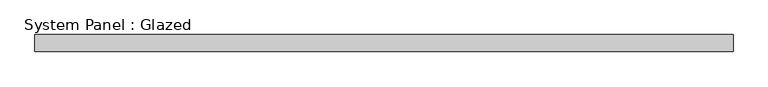
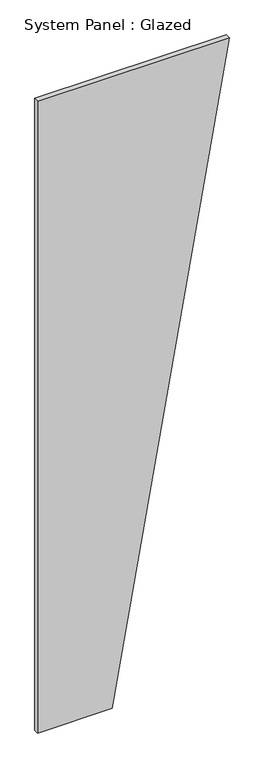
"""IFC4 building model written with IfcOpenShell, lengths in millimetres: plate geometry, System Panel : Glazed."""

import ifcopenshell
import ifcopenshell.guid

model = None  # the IFC model being written
_history = None  # IfcOwnerHistory: only IFC2X3 demands one
_inside = {}  # id of a spatial element -> (the spatial element, [elements in it])
_under = {}  # id of a project, library or spatial element -> (it, [spatial elements below it])
_declared = {}  # id of a project -> (the project, [libraries it declares])
_typed = {}  # id of a type object -> (the type object, [elements of that type])
_made_of = {}  # id of a material, layer set ... -> (it, [elements and type objects made of it])


def new_model(schema):
    """Start an empty IFC model of exactly this schema.

    Asked for "IFC4X3", IfcOpenShell would pick the latest addendum, in which some entities
    have other attributes; the version numbers below select the first issue.
    IFC2X3 requires an IfcOwnerHistory on every rooted entity: one is made here for all.
    """
    global model, _history
    if schema == "IFC4X3":
        model = ifcopenshell.file(schema_version=(4, 3, 0, 0))
    else:
        model = ifcopenshell.file(schema=schema)
    _inside.clear()
    _under.clear()
    _declared.clear()
    _typed.clear()
    _made_of.clear()
    _history = None
    if model.schema == "IFC2X3":
        org = make("IfcOrganization", Name="unknown")
        user = make(
            "IfcPersonAndOrganization",
            ThePerson=make("IfcPerson", FamilyName="unknown"),
            TheOrganization=org,
        )
        app = make(
            "IfcApplication",
            ApplicationDeveloper=org,
            Version="unknown",
            ApplicationFullName="unknown",
            ApplicationIdentifier="unknown",
        )
        _history = make(
            "IfcOwnerHistory",
            OwningUser=user,
            OwningApplication=app,
            ChangeAction="ADDED",
            CreationDate=0,
        )
    return model


def make(cls, **values):
    """One entity of the class cls with the attributes given. An attribute that is None is left unset."""
    return model.create_entity(
        cls, **{name: value for name, value in values.items() if value is not None}
    )


def rooted(cls, **values):
    """An entity with a GlobalId (a new one), such as an element, a storey or a relation."""
    return make(cls, GlobalId=ifcopenshell.guid.new(), OwnerHistory=_history, **values)


def si_unit(unit_type, name, prefix=None):
    """IfcSIUnit, for example si_unit("LENGTHUNIT", "METRE", prefix="MILLI")."""
    return make("IfcSIUnit", UnitType=unit_type, Prefix=prefix, Name=name)


def assignment(units):
    """IfcUnitAssignment: the units of a project."""
    return None if units is None else make("IfcUnitAssignment", Units=units)


def point(xyz):
    """IfcCartesianPoint."""
    return None if xyz is None else make("IfcCartesianPoint", Coordinates=xyz)


def direction(xyz):
    """IfcDirection."""
    return None if xyz is None else make("IfcDirection", DirectionRatios=xyz)


def frame(location, z_axis=None, x_axis=None):
    """IfcAxis2Placement3D, a coordinate frame: its origin and axes. An axis left out is left unset."""
    return make(
        "IfcAxis2Placement3D",
        Location=point(location),
        Axis=direction(z_axis),
        RefDirection=direction(x_axis),
    )


def origin():
    """The frame at (0, 0, 0) with its axes left unset."""
    return frame((0.0, 0.0, 0.0))


def place(relative_to, where):
    """IfcLocalPlacement: puts the frame where relative to a parent placement (None: the world)."""
    return make(
        "IfcLocalPlacement", PlacementRelTo=relative_to, RelativePlacement=where
    )


def context(
    kind, dimensions, precision=None, world=None, true_north=None, identifier=None
):
    """IfcGeometricRepresentationContext, for example the 3D "Model" context."""
    return make(
        "IfcGeometricRepresentationContext",
        ContextIdentifier=identifier,
        ContextType=kind,
        CoordinateSpaceDimension=dimensions,
        Precision=precision,
        WorldCoordinateSystem=world,
        TrueNorth=true_north,
    )


def project(units=None, contexts=None):
    """IfcProject with its units and contexts."""
    return rooted(
        "IfcProject",
        Name="project",
        RepresentationContexts=contexts,
        UnitsInContext=assignment(units),
    )


def spatial(cls, under=None, at=None, **own):
    """A site, building, storey or space (cls), placed at a placement, below another one or the project."""
    s = rooted(cls, ObjectPlacement=at, **own)
    if under is not None:
        _under.setdefault(under.id(), (under, []))[1].append(s)
    return s


def polyline(points):
    """IfcPolyline through the points."""
    return make("IfcPolyline", Points=[point(p) for p in points])


def outline(outer, holes=None, kind="AREA"):
    """IfcArbitraryClosedProfileDef: a profile drawn as a closed curve; with holes, ...WithVoids."""
    if holes is None:
        return make("IfcArbitraryClosedProfileDef", ProfileType=kind, OuterCurve=outer)
    return make(
        "IfcArbitraryProfileDefWithVoids",
        ProfileType=kind,
        OuterCurve=outer,
        InnerCurves=holes,
    )


def extrude(swept, where, along, depth):
    """IfcExtrudedAreaSolid: the profile swept, set in the frame where, extruded along a direction by depth."""
    return make(
        "IfcExtrudedAreaSolid",
        SweptArea=swept,
        Position=where,
        ExtrudedDirection=direction(along),
        Depth=depth,
    )


def shape(context_of_items, identifier, shape_type, items):
    """IfcShapeRepresentation: the items that make up one representation, for example the "Body"."""
    return make(
        "IfcShapeRepresentation",
        ContextOfItems=context_of_items,
        RepresentationIdentifier=identifier,
        RepresentationType=shape_type,
        Items=items,
    )


def source(mapping_origin, context_of_items, identifier, shape_type, items):
    """IfcRepresentationMap: a shape defined once, which mapped items show again and again."""
    return make(
        "IfcRepresentationMap",
        MappingOrigin=mapping_origin,
        MappedRepresentation=shape(context_of_items, identifier, shape_type, items),
    )


def transform(
    local_origin,
    x_axis=None,
    y_axis=None,
    z_axis=None,
    scale=None,
    scale2=None,
    scale3=None,
    uniform=True,
):
    """IfcCartesianTransformationOperator3D, or its non-uniform kind. x_axis, y_axis, z_axis: its Axis1, 2, 3."""
    if uniform:
        return make(
            "IfcCartesianTransformationOperator3D",
            Axis1=direction(x_axis),
            Axis2=direction(y_axis),
            LocalOrigin=point(local_origin),
            Scale=scale,
            Axis3=direction(z_axis),
        )
    return make(
        "IfcCartesianTransformationOperator3DnonUniform",
        Axis1=direction(x_axis),
        Axis2=direction(y_axis),
        LocalOrigin=point(local_origin),
        Scale=scale,
        Axis3=direction(z_axis),
        Scale2=scale2,
        Scale3=scale3,
    )


def mapped(mapping_source, mapping_target):
    """IfcMappedItem: shows the shape of a source again, moved by a transform."""
    return make(
        "IfcMappedItem", MappingSource=mapping_source, MappingTarget=mapping_target
    )


def made_of(thing, what):
    """Note that an element or type object is made of a material, layer set ...; save() writes the relation."""
    if what is not None:
        _made_of.setdefault(what.id(), (what, []))[1].append(thing)
    return thing


def element(
    cls,
    number,
    at=None,
    inside=None,
    cuts=None,
    type_object=None,
    material=None,
    context=None,
    identifier="Body",
    shape_type=None,
    held_by="IfcProductDefinitionShape",
    body=None,
    shapes=None,
    **own,
):
    """One element of the class cls, such as IfcWall. Its Tag is "e" and its number.

    at: its placement. inside: the storey or other place that contains it. cuts: it is an
    opening in that element (IfcRelVoidsElement). A single representation is given by context,
    identifier, shape_type and body (its items); several are given by shapes. held_by: the class
    of the entity that holds the representations. save() writes the other relations.
    """
    e = rooted(cls, Tag="e%d" % number, ObjectPlacement=at, **own)
    if body is not None:
        shapes = [shape(context, identifier, shape_type, body)]
    if shapes is not None:
        e.Representation = make(held_by, Representations=shapes)
    if inside is not None:
        _inside.setdefault(inside.id(), (inside, []))[1].append(e)
    if cuts is not None:
        rooted(
            "IfcRelVoidsElement", RelatingBuildingElement=cuts, RelatedOpeningElement=e
        )
    if type_object is not None:
        _typed.setdefault(type_object.id(), (type_object, []))[1].append(e)
    return made_of(e, material)


def aggregate(whole, parts):
    """IfcRelAggregates: a whole, such as a stair, and the parts it consists of."""
    return rooted("IfcRelAggregates", RelatingObject=whole, RelatedObjects=parts)


def save(model, path):
    """Write the relations noted so far, then the file.

    IfcRelAggregates (storeys below a building ...), IfcRelContainedInSpatialStructure (elements
    in a storey), IfcRelDefinesByType, IfcRelAssociatesMaterial and IfcRelDeclares: one each for
    every whole, place, type object, material and project.
    """
    for whole, parts in _under.values():
        aggregate(whole, parts)
    for where, things in _inside.values():
        rooted(
            "IfcRelContainedInSpatialStructure",
            RelatedElements=things,
            RelatingStructure=where,
        )
    for kind, things in _typed.values():
        rooted("IfcRelDefinesByType", RelatedObjects=things, RelatingType=kind)
    for what, things in _made_of.values():
        rooted("IfcRelAssociatesMaterial", RelatedObjects=things, RelatingMaterial=what)
    for by, libraries in _declared.values():
        rooted("IfcRelDeclares", RelatingContext=by, RelatedDefinitions=libraries)
    model.write(path)


def system_panel_glazed_ce152239(model_context):
    return source(origin(), model_context, "Body", "SweptSolid", [
        extrude(outline(polyline([(0.0, -525.4711374), (0.0, -117.0082603), (3657.6, 525.4711374), (3657.6, -525.4711374), (0.0, -525.4711374)])), frame((0.0, -44.45, 0.0), z_axis=(0.0, 1.0, 0.0), x_axis=(0.0, 0.0, 1.0)), (0.0, 0.0, 1.0), 25.4),
    ])


if __name__ == "__main__":
    model = new_model("IFC4")
    model_context = context("Model", 3, world=origin())
    ifc_project = project(units=[si_unit("LENGTHUNIT", "METRE", prefix="MILLI")], contexts=[model_context])
    site = spatial("IfcSite", under=ifc_project)
    building = spatial("IfcBuilding", under=site)
    placement = place(None, origin())
    system_panel_glazed_shape = system_panel_glazed_ce152239(model_context)
    element("IfcPlate", 1, ObjectType="System Panel : Glazed", at=placement, inside=building, context=model_context, shape_type="MappedRepresentation", body=[
        mapped(system_panel_glazed_shape, transform((0.0, 0.0, 0.0), x_axis=(1.0, 0.0, 0.0), y_axis=(0.0, 1.0, 0.0), z_axis=(0.0, 0.0, 1.0))),
    ])
    save(model, "model.ifc")

# Revit data of these elements
# Type "System Panel : Glazed"
#   Construction Type Id = "GSP4R"
#   Analytic Construction = "1/8 in Pilkington single glazing"
#   Visual Light Transmittance = 0.9
#   Solar Heat Gain Coefficient = 0.86
#   Heat Transfer Coefficient (U) = 1.18115 BTU/(h·ft²·°F)
#   Define Thermal Properties by = 1
# Element 1 (IfcPlate, "System Panel : Glazed")
#   Materials on its faces: "Glass"
# Materials
#   "Glass": class "Glass", colour RGB 0 128 192, transparency 0.75, Description = "Soda Lime Glass", Cost = 0
